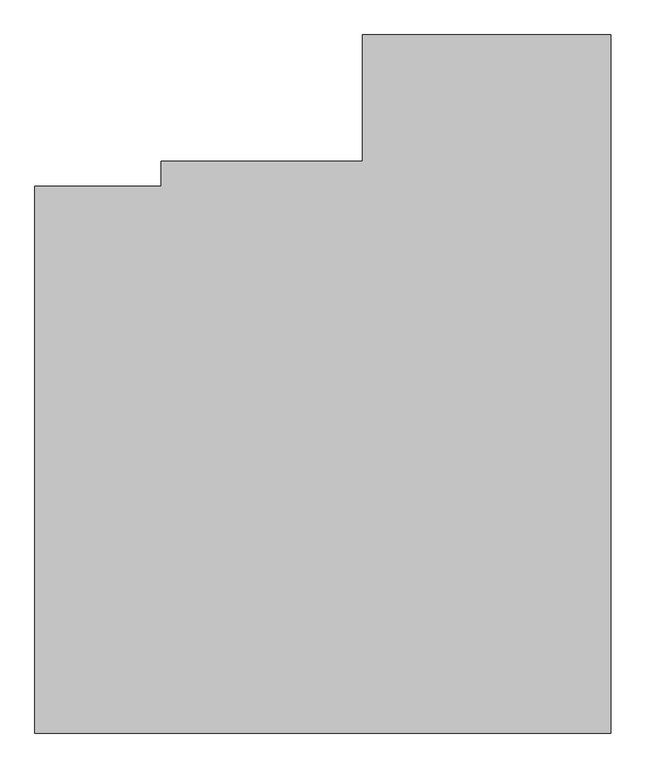
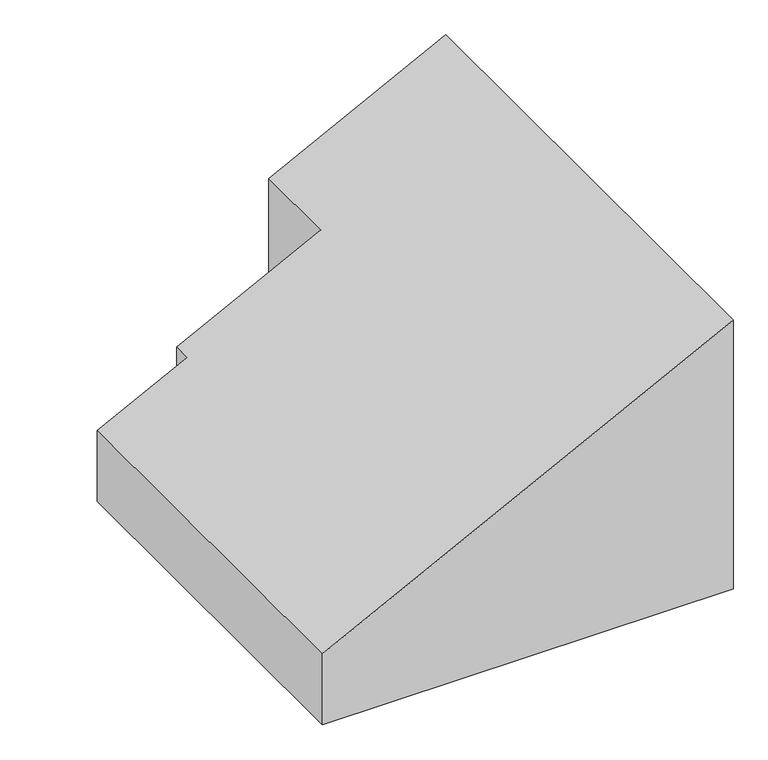
"""IFC4 building model written with IfcOpenShell, lengths in millimetres: proxy geometry, 0_3d."""

from ifc_helpers import new_model, si_unit, origin, place, context, project, spatial, faceted_brep, source, transform, mapped, element, save


def generic_models_fb7019a2(model_context):
    return source(origin(), model_context, "Body", "Brep", [
        faceted_brep([(4680.0, 5670.0, 3237.913011), (2664.6018366, 5670.0, 2211.0163558), (2664.6018366, 4645.0, 2211.0163558), (1025.0, 4645.0, 1375.5974931), (1025.0, 4440.2642941, 1375.5974931), (0.0, 4440.2642941, 853.3339073), (0.0, 0.0, 853.3339073), (4680.0, 0.0, 3237.913011), (1025.0, 4440.2642941, 0.0), (0.0, 4440.2642941, 0.0), (1025.0, 4645.0, 0.0), (2664.6018366, 4645.0, 0.0), (2664.6018366, 5670.0, 0.0), (4680.0, 5670.0, 0.0), (4680.0, 0.0, 0.0), (0.0, 0.0, 0.0)], [[[0, 1, 2, 3, 4, 5, 6, 7]], [[5, 4, 8, 9]], [[4, 3, 10, 8]], [[3, 2, 11, 10]], [[2, 1, 12, 11]], [[1, 0, 13, 12]], [[14, 13, 0, 7]], [[7, 6, 15, 14]], [[6, 5, 9, 15]], [[11, 12, 13, 14, 15, 9, 8, 10]]]),
    ])


if __name__ == "__main__":
    model = new_model("IFC4")
    model_context = context("Model", 3, world=origin())
    ifc_project = project(units=[si_unit("LENGTHUNIT", "METRE", prefix="MILLI")], contexts=[model_context])
    site = spatial("IfcSite", under=ifc_project)
    building = spatial("IfcBuilding", under=site)
    placement = place(None, origin())
    generic_models_shape = generic_models_fb7019a2(model_context)
    element("IfcBuildingElementProxy", 1, Name="0_3d", ObjectType="0_3d", at=placement, inside=building, context=model_context, shape_type="MappedRepresentation", body=[
        mapped(generic_models_shape, transform((0.0, 0.0, 0.0), x_axis=(1.0, 0.0, 0.0), y_axis=(0.0, 1.0, 0.0), z_axis=(0.0, 0.0, 1.0))),
    ])
    save(model, "model.ifc")

# Revit data of these elements
# Element 1 (IfcBuildingElementProxy, "0_3d")
#   Materials on its faces: "*1"
# Materials
#   "*1": class "Unassigned", colour RGB 175 175 175, transparency 0
